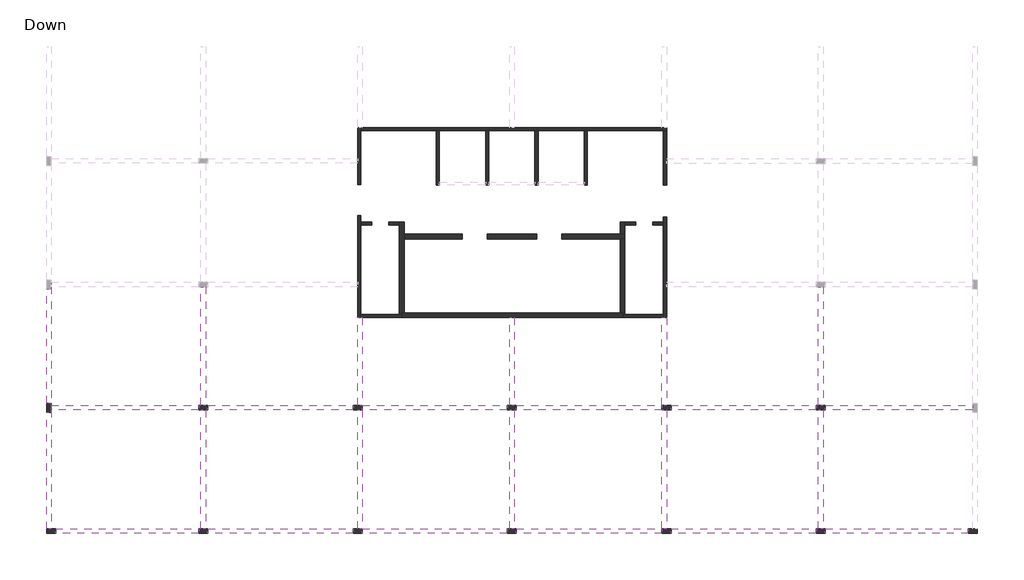
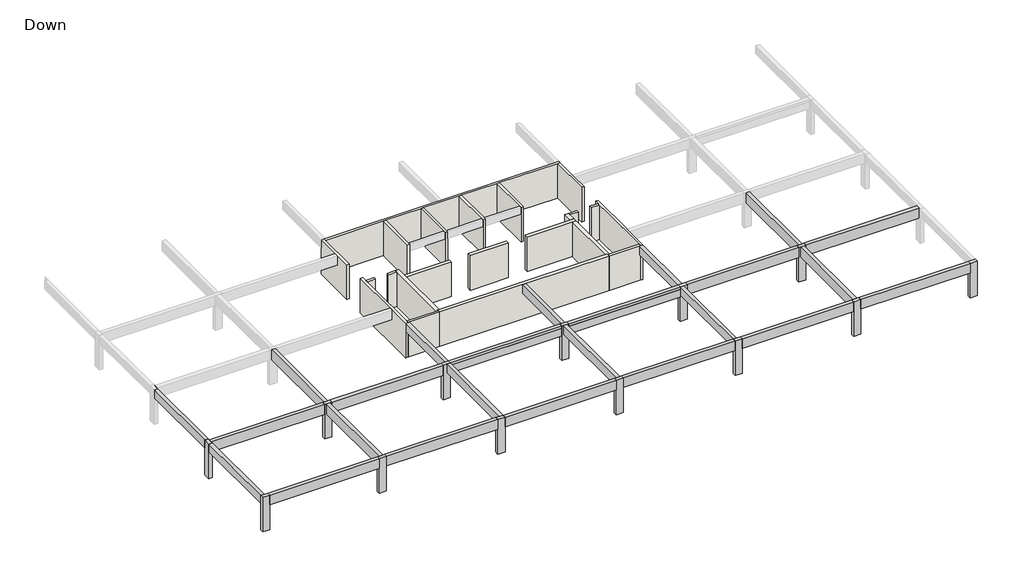
# One storey, part 1 of 2: 24 beams, 22 walls, 13 columns.
# Revit data of these elements (continued)
# Project information (continued)
#   Project Name = "Project 023"
#   Project Number = "מספר פרויקט"
# Type "Concrete Rectengular Beam : 30/70"
#   Length [instance default] = 152.4 cm
#   b = 30 cm
#   h = 70 cm
#   Structural Material [instance default] = Concrete
#   Assembly Code = ""
# Type "Concrete Rectengular Beam : 30/75"
#   Length [instance default] = 152.4 cm
#   b = 30 cm
#   h = 75 cm
#   Structural Material [instance default] = Concrete
#   Assembly Code = ""
# Type "Concrete Rectengular Beam : 30/85"
#   Length [instance default] = 152.4 cm
#   b = 30 cm
#   h = 85 cm
#   Structural Material [instance default] = Concrete
#   Assembly Code = ""
# Type "Concrete Rectengular Beam : 30/90"
#   Length [instance default] = 152.4 cm
#   b = 30 cm
#   h = 90 cm
#   Structural Material [instance default] = Concrete
#   Assembly Code = ""
# Type "Concrete Rectengular Column : 30/60"
#   b = 30 cm
#   h = 60 cm
#   Structural Material [instance default] = Concrete
# Type "20"
#   Layers, outside or top first: 20 cm "Concrete" (function 1)
# Type "30"
#   Layers, outside or top first: 30 cm "Concrete" (function 1)
# Element 1 (IfcBeam, "Concrete Rectengular Beam : 30/70")
#   Comments = ""
#   Mark = "B9"
#   SOFiSTiK_AMG_Comments = ""
#   SOFiSTiK_AMG_Scheduled = yes
#   SOFiSTiK_AMG_Adjusted = yes
#   Structural Material = Concrete
#   Phase Created = New Construction
#   Materials on its faces: "Concrete"
# Element 2 (IfcBeam, "Concrete Rectengular Beam : 30/70")
#   Comments = ""
#   Mark = "B10"
#   SOFiSTiK_AMG_Comments = ""
#   SOFiSTiK_AMG_Scheduled = yes
#   SOFiSTiK_AMG_Adjusted = yes
#   Structural Material = Concrete
#   Phase Created = New Construction
#   Materials on its faces: "Concrete"
# Element 3 (IfcBeam, "Concrete Rectengular Beam : 30/75")
#   Comments = ""
#   Mark = "B20"
#   SOFiSTiK_AMG_Comments = ""
#   SOFiSTiK_AMG_Scheduled = yes
#   SOFiSTiK_AMG_Adjusted = yes
#   Structural Material = Concrete
#   Phase Created = New Construction
#   Materials on its faces: "Concrete"
# Element 4 (IfcBeam, "Concrete Rectengular Beam : 30/75")
#   Comments = ""
#   Mark = "B21"
#   SOFiSTiK_AMG_Comments = ""
#   SOFiSTiK_AMG_Scheduled = yes
#   SOFiSTiK_AMG_Adjusted = yes
#   Structural Material = Concrete
#   Phase Created = New Construction
#   Materials on its faces: "Concrete"
# Element 5 (IfcBeam, "Concrete Rectengular Beam : 30/75")
#   Comments = ""
#   Mark = "B22"
#   SOFiSTiK_AMG_Comments = ""
#   SOFiSTiK_AMG_Scheduled = yes
#   SOFiSTiK_AMG_Adjusted = yes
#   Structural Material = Concrete
#   Phase Created = New Construction
#   Materials on its faces: "Concrete"
# Element 6 (IfcBeam, "Concrete Rectengular Beam : 30/75")
#   Comments = ""
#   Mark = "B23"
#   SOFiSTiK_AMG_Comments = ""
#   SOFiSTiK_AMG_Scheduled = yes
#   SOFiSTiK_AMG_Adjusted = yes
#   Structural Material = Concrete
#   Phase Created = New Construction
#   Materials on its faces: "Concrete"
# Element 7 (IfcBeam, "Concrete Rectengular Beam : 30/75")
#   Comments = ""
#   Mark = "B24"
#   SOFiSTiK_AMG_Comments = ""
#   SOFiSTiK_AMG_Scheduled = yes
#   SOFiSTiK_AMG_Adjusted = yes
#   Structural Material = Concrete
#   Phase Created = New Construction
#   Materials on its faces: "Concrete"
# Element 8 (IfcBeam, "Concrete Rectengular Beam : 30/75")
#   Comments = ""
#   Mark = "B25"
#   SOFiSTiK_AMG_Comments = ""
#   SOFiSTiK_AMG_Scheduled = yes
#   SOFiSTiK_AMG_Adjusted = yes
#   Structural Material = Concrete
#   Phase Created = New Construction
#   Materials on its faces: "Concrete"
# Element 9 (IfcBeam, "Concrete Rectengular Beam : 30/85")
#   Comments = ""
#   Mark = "B32"
#   SOFiSTiK_AMG_Comments = ""
#   SOFiSTiK_AMG_Scheduled = yes
#   SOFiSTiK_AMG_Adjusted = yes
#   Structural Material = Concrete
#   Phase Created = New Construction
#   Materials on its faces: "Concrete"
# Element 10 (IfcBeam, "Concrete Rectengular Beam : 30/85")
#   Comments = ""
#   Mark = "B33"
#   SOFiSTiK_AMG_Comments = ""
#   SOFiSTiK_AMG_Scheduled = yes
#   SOFiSTiK_AMG_Adjusted = yes
#   Structural Material = Concrete
#   Phase Created = New Construction
#   Materials on its faces: "Concrete"
# Element 11 (IfcBeam, "Concrete Rectengular Beam : 30/85")
#   Comments = ""
#   Mark = "B34"
#   SOFiSTiK_AMG_Comments = ""
#   SOFiSTiK_AMG_Scheduled = yes
#   SOFiSTiK_AMG_Adjusted = yes
#   Structural Material = Concrete
#   Phase Created = New Construction
#   Materials on its faces: "Concrete"
# Element 12 (IfcBeam, "Concrete Rectengular Beam : 30/85")
#   Comments = ""
#   Mark = "B35"
#   SOFiSTiK_AMG_Comments = ""
#   SOFiSTiK_AMG_Scheduled = yes
#   SOFiSTiK_AMG_Adjusted = yes
#   Structural Material = Concrete
#   Phase Created = New Construction
#   Materials on its faces: "Concrete"
# Element 13 (IfcBeam, "Concrete Rectengular Beam : 30/85")
#   Comments = ""
#   Mark = "B36"
#   SOFiSTiK_AMG_Comments = ""
#   SOFiSTiK_AMG_Scheduled = yes
#   SOFiSTiK_AMG_Adjusted = yes
#   Structural Material = Concrete
#   Phase Created = New Construction
#   Materials on its faces: "Concrete"
# Element 14 (IfcBeam, "Concrete Rectengular Beam : 30/85")
#   Comments = ""
#   Mark = "B37"
#   SOFiSTiK_AMG_Comments = ""
#   SOFiSTiK_AMG_Scheduled = yes
#   SOFiSTiK_AMG_Adjusted = yes
#   Structural Material = Concrete
#   Phase Created = New Construction
#   Materials on its faces: "Concrete"
# Element 15 (IfcBeam, "Concrete Rectengular Beam : 30/90")
#   Comments = ""
#   Mark = "B46"
#   SOFiSTiK_AMG_Comments = ""
#   SOFiSTiK_AMG_Scheduled = yes
#   SOFiSTiK_AMG_Adjusted = yes
#   Structural Material = Concrete
#   Phase Created = New Construction
#   Materials on its faces: "Concrete"
# Element 16 (IfcBeam, "Concrete Rectengular Beam : 30/90")
#   Comments = ""
#   Mark = "B47"
#   SOFiSTiK_AMG_Comments = ""
#   SOFiSTiK_AMG_Scheduled = yes
#   SOFiSTiK_AMG_Adjusted = yes
#   Structural Material = Concrete
#   Phase Created = New Construction
#   Materials on its faces: "Concrete"
# Element 17 (IfcBeam, "Concrete Rectengular Beam : 30/90")
#   Comments = ""
#   Mark = "B48"
#   SOFiSTiK_AMG_Comments = ""
#   SOFiSTiK_AMG_Scheduled = yes
#   SOFiSTiK_AMG_Adjusted = yes
#   Structural Material = Concrete
#   Phase Created = New Construction
#   Materials on its faces: "Concrete"
# Element 18 (IfcBeam, "Concrete Rectengular Beam : 30/90")
#   Comments = ""
#   Mark = "B49"
#   SOFiSTiK_AMG_Comments = ""
#   SOFiSTiK_AMG_Scheduled = yes
#   SOFiSTiK_AMG_Adjusted = yes
#   Structural Material = Concrete
#   Phase Created = New Construction
#   Materials on its faces: "Concrete"
# Element 19 (IfcBeam, "Concrete Rectengular Beam : 30/90")
#   Comments = ""
#   Mark = "B50"
#   SOFiSTiK_AMG_Comments = ""
#   SOFiSTiK_AMG_Scheduled = yes
#   SOFiSTiK_AMG_Adjusted = yes
#   Structural Material = Concrete
#   Phase Created = New Construction
#   Materials on its faces: "Concrete"
# Element 20 (IfcBeam, "Concrete Rectengular Beam : 30/90")
#   Comments = ""
#   Mark = "B51"
#   SOFiSTiK_AMG_Comments = ""
#   SOFiSTiK_AMG_Scheduled = yes
#   SOFiSTiK_AMG_Adjusted = yes
#   Structural Material = Concrete
#   Phase Created = New Construction
#   Materials on its faces: "Concrete"
# Element 21 (IfcBeam, "Concrete Rectengular Beam : 30/90")
#   Comments = ""
#   Mark = "B61"
#   SOFiSTiK_AMG_Comments = ""
#   SOFiSTiK_AMG_Scheduled = yes
#   SOFiSTiK_AMG_Adjusted = yes
#   Structural Material = Concrete
#   Phase Created = New Construction
#   Materials on its faces: "Concrete"
# Element 22 (IfcBeam, "Concrete Rectengular Beam : 30/90")
#   Comments = ""
#   Mark = "B62"
#   SOFiSTiK_AMG_Comments = ""
#   SOFiSTiK_AMG_Scheduled = yes
#   SOFiSTiK_AMG_Adjusted = yes
#   Structural Material = Concrete
#   Phase Created = New Construction
#   Materials on its faces: "Concrete"
# Element 23 (IfcBeam, "Concrete Rectengular Beam : 30/90")
#   Comments = ""
#   Mark = "B66"
#   SOFiSTiK_AMG_Comments = ""
#   SOFiSTiK_AMG_Scheduled = yes
#   SOFiSTiK_AMG_Adjusted = yes
#   Structural Material = Concrete
#   Phase Created = New Construction
#   Materials on its faces: "Concrete"
# Element 24 (IfcBeam, "Concrete Rectengular Beam : 30/90")
#   Comments = ""
#   Mark = "B67"
#   SOFiSTiK_AMG_Comments = ""
#   SOFiSTiK_AMG_Scheduled = yes
#   SOFiSTiK_AMG_Adjusted = yes
#   Structural Material = Concrete
#   Phase Created = New Construction
#   Materials on its faces: "Concrete"
# Element 25 (IfcColumn, "Concrete Rectengular Column : 30/60")
#   Comments = ""
#   Mark = "C3"
#   SOFiSTiK_AMG_Comments = ""
#   SOFiSTiK_AMG_Scheduled = yes
#   SOFiSTiK_AMG_Adjusted = yes
#   Structural Material = Concrete
#   Phase Created = New Construction
#   Materials on its faces: "Concrete"
# Element 26 (IfcColumn, "Concrete Rectengular Column : 30/60")
#   Comments = ""
#   Mark = "C7"
#   SOFiSTiK_AMG_Comments = ""
#   SOFiSTiK_AMG_Scheduled = yes
#   SOFiSTiK_AMG_Adjusted = yes
#   Structural Material = Concrete
#   Phase Created = New Construction
#   Materials on its faces: "Concrete"
# Element 27 (IfcColumn, "Concrete Rectengular Column : 30/60")
#   Comments = ""
#   Mark = "C8"
#   SOFiSTiK_AMG_Comments = ""
#   SOFiSTiK_AMG_Scheduled = yes
#   SOFiSTiK_AMG_Adjusted = yes
#   Structural Material = Concrete
#   Phase Created = New Construction
#   Materials on its faces: "Concrete"
# Element 28 (IfcColumn, "Concrete Rectengular Column : 30/60")
#   Comments = ""
#   Mark = "C14"
#   SOFiSTiK_AMG_Comments = ""
#   SOFiSTiK_AMG_Scheduled = yes
#   SOFiSTiK_AMG_Adjusted = yes
#   Structural Material = Concrete
#   Phase Created = New Construction
#   Materials on its faces: "Concrete"
# Element 29 (IfcColumn, "Concrete Rectengular Column : 30/60")
#   Comments = ""
#   Mark = "C15"
#   SOFiSTiK_AMG_Comments = ""
#   SOFiSTiK_AMG_Scheduled = yes
#   SOFiSTiK_AMG_Adjusted = yes
#   Structural Material = Concrete
#   Phase Created = New Construction
#   Materials on its faces: "Concrete"
# Element 30 (IfcColumn, "Concrete Rectengular Column : 30/60")
#   Comments = ""
#   Mark = "C17"
#   SOFiSTiK_AMG_Comments = ""
#   SOFiSTiK_AMG_Scheduled = yes
#   SOFiSTiK_AMG_Adjusted = yes
#   Structural Material = Concrete
#   Phase Created = New Construction
#   Materials on its faces: "Concrete"
# Element 31 (IfcColumn, "Concrete Rectengular Column : 30/60")
#   Comments = ""
#   Mark = "C23"
#   SOFiSTiK_AMG_Comments = ""
#   SOFiSTiK_AMG_Scheduled = yes
#   SOFiSTiK_AMG_Adjusted = yes
#   Structural Material = Concrete
#   Phase Created = New Construction
#   Materials on its faces: "Concrete"
# Element 32 (IfcColumn, "Concrete Rectengular Column : 30/60")
#   Comments = ""
#   Mark = "C24"
#   SOFiSTiK_AMG_Comments = ""
#   SOFiSTiK_AMG_Scheduled = yes
#   SOFiSTiK_AMG_Adjusted = yes
#   Structural Material = Concrete
#   Phase Created = New Construction
#   Materials on its faces: "Concrete"
# Element 33 (IfcColumn, "Concrete Rectengular Column : 30/60")
#   Comments = ""
#   Mark = "C25"
#   SOFiSTiK_AMG_Comments = ""
#   SOFiSTiK_AMG_Scheduled = yes
#   SOFiSTiK_AMG_Adjusted = yes
#   Structural Material = Concrete
#   Phase Created = New Construction
#   Materials on its faces: "Concrete"
# Element 34 (IfcColumn, "Concrete Rectengular Column : 30/60")
#   Comments = ""
#   Mark = "C26"
#   SOFiSTiK_AMG_Comments = ""
#   SOFiSTiK_AMG_Scheduled = yes
#   SOFiSTiK_AMG_Adjusted = yes
#   Structural Material = Concrete
#   Phase Created = New Construction
#   Materials on its faces: "Concrete"
# Element 35 (IfcColumn, "Concrete Rectengular Column : 30/60")
#   Comments = ""
#   Mark = "C27"
#   SOFiSTiK_AMG_Comments = ""
#   SOFiSTiK_AMG_Scheduled = yes
#   SOFiSTiK_AMG_Adjusted = yes
#   Structural Material = Concrete
#   Phase Created = New Construction
#   Materials on its faces: "Concrete"
# Element 36 (IfcColumn, "Concrete Rectengular Column : 30/60")
#   Comments = ""
#   Mark = "C35"
#   SOFiSTiK_AMG_Comments = ""
#   SOFiSTiK_AMG_Scheduled = yes
#   SOFiSTiK_AMG_Adjusted = yes
#   Structural Material = Concrete
#   Phase Created = New Construction
#   Materials on its faces: "Concrete"
# Element 37 (IfcColumn, "Concrete Rectengular Column : 30/60")
#   Comments = ""
#   Mark = "C36"
#   SOFiSTiK_AMG_Comments = ""
#   SOFiSTiK_AMG_Scheduled = yes
#   SOFiSTiK_AMG_Adjusted = yes
#   Structural Material = Concrete
#   Phase Created = New Construction
#   Materials on its faces: "Concrete"
# Element 38 (IfcWall, "20")
#   Comments = ""
#   Mark = "W1"
#   SOFiSTiK_EdgeZones = "W1"
#   SOFiSTiK_AMG_Comments = ""
#   Top Offset = 0 cm
#   Base Offset = 0 cm
#   wall height = 308 cm
#   SOFiSTiK_AMG_Scheduled = yes
#   SOFiSTiK_AMG_Adjusted = yes
#   Phase Created = New Construction
#   Base Constraint = Down
#   Top Constraint = Typical Floor
#   Materials on its faces: "Concrete"
# Element 39 (IfcWall, "20")
#   Comments = ""
#   Mark = "W2"
#   SOFiSTiK_EdgeZones = "W2"
#   SOFiSTiK_AMG_Comments = ""
#   Top Offset = 0 cm
#   Base Offset = 0 cm
#   wall height = 308 cm
#   SOFiSTiK_AMG_Scheduled = yes
#   SOFiSTiK_AMG_Adjusted = yes
#   Phase Created = New Construction
#   Base Constraint = Down
#   Top Constraint = Typical Floor
#   Materials on its faces: "Concrete"
# Element 40 (IfcWall, "20")
#   Comments = ""
#   Mark = "W3"
#   SOFiSTiK_EdgeZones = "W3"
#   SOFiSTiK_AMG_Comments = ""
#   Top Offset = 0 cm
#   Base Offset = 0 cm
#   wall height = 308 cm
#   SOFiSTiK_AMG_Scheduled = yes
#   SOFiSTiK_AMG_Adjusted = yes
#   Phase Created = New Construction
#   Base Constraint = Down
#   Top Constraint = Typical Floor
#   Materials on its faces: "Concrete"
# Element 41 (IfcWall, "20")
#   Comments = ""
#   Mark = "W4"
#   SOFiSTiK_EdgeZones = "W4"
#   SOFiSTiK_AMG_Comments = ""
#   Top Offset = 0 cm
#   Base Offset = 0 cm
#   wall height = 308 cm
#   SOFiSTiK_AMG_Scheduled = yes
#   SOFiSTiK_AMG_Adjusted = yes
#   Phase Created = New Construction
#   Base Constraint = Down
#   Top Constraint = Typical Floor
#   Materials on its faces: "Concrete"
# Element 42 (IfcWall, "20")
#   Comments = ""
#   Mark = "W5"
#   SOFiSTiK_EdgeZones = "W5"
#   SOFiSTiK_AMG_Comments = ""
#   Top Offset = 0 cm
#   Base Offset = 0 cm
#   wall height = 308 cm
#   SOFiSTiK_AMG_Scheduled = yes
#   SOFiSTiK_AMG_Adjusted = yes
#   Phase Created = New Construction
#   Base Constraint = Down
#   Top Constraint = Typical Floor
#   Materials on its faces: "Concrete"
# Element 43 (IfcWall, "20")
#   Comments = ""
#   Mark = "W6"
#   SOFiSTiK_EdgeZones = "W6"
#   SOFiSTiK_AMG_Comments = ""
#   Top Offset = 0 cm
#   Base Offset = 0 cm
#   wall height = 308 cm
#   SOFiSTiK_AMG_Scheduled = yes
#   SOFiSTiK_AMG_Adjusted = yes
#   Phase Created = New Construction
#   Base Constraint = Down
#   Top Constraint = Typical Floor
#   Materials on its faces: "Concrete"
# Element 44 (IfcWall, "20")
#   Comments = ""
#   Mark = "W7"
#   SOFiSTiK_EdgeZones = "W7"
#   SOFiSTiK_AMG_Comments = ""
#   Top Offset = 0 cm
#   Base Offset = 0 cm
#   wall height = 308 cm
#   SOFiSTiK_AMG_Scheduled = yes
#   SOFiSTiK_AMG_Adjusted = yes
#   Phase Created = New Construction
#   Base Constraint = Down
#   Top Constraint = Typical Floor
#   Materials on its faces: "Concrete"
# Element 45 (IfcWall, "20")
#   Comments = ""
#   Mark = "W8"
#   SOFiSTiK_EdgeZones = "W8"
#   SOFiSTiK_AMG_Comments = ""
#   Top Offset = 0 cm
#   Base Offset = 0 cm
#   wall height = 308 cm
#   SOFiSTiK_AMG_Scheduled = yes
#   SOFiSTiK_AMG_Adjusted = yes
#   Phase Created = New Construction
#   Base Constraint = Down
#   Top Constraint = Typical Floor
#   Materials on its faces: "Concrete"
# Element 46 (IfcWall, "20")
#   Comments = ""
#   Mark = "W9"
#   SOFiSTiK_EdgeZones = "W9"
#   SOFiSTiK_AMG_Comments = ""
#   Top Offset = 0 cm
#   Base Offset = 0 cm
#   wall height = 308 cm
#   SOFiSTiK_AMG_Scheduled = yes
#   SOFiSTiK_AMG_Adjusted = yes
#   Phase Created = New Construction
#   Base Constraint = Down
#   Top Constraint = Typical Floor
#   Materials on its faces: "Concrete"
# Element 47 (IfcWall, "20")
#   Comments = ""
#   Mark = "W10"
#   SOFiSTiK_EdgeZones = "W10"
#   SOFiSTiK_AMG_Comments = ""
#   Top Offset = 0 cm
#   Base Offset = 0 cm
#   wall height = 308 cm
#   SOFiSTiK_AMG_Scheduled = yes
#   SOFiSTiK_AMG_Adjusted = yes
#   Phase Created = New Construction
#   Base Constraint = Down
#   Top Constraint = Typical Floor
#   Materials on its faces: "Concrete"
# Element 48 (IfcWall, "20")
#   Comments = ""
#   Mark = "W11"
#   SOFiSTiK_EdgeZones = "W11"
#   SOFiSTiK_AMG_Comments = ""
#   Top Offset = 0 cm
#   Base Offset = 0 cm
#   wall height = 308 cm
#   SOFiSTiK_AMG_Scheduled = yes
#   SOFiSTiK_AMG_Adjusted = yes
#   Phase Created = New Construction
#   Base Constraint = Down
#   Top Constraint = Typical Floor
#   Materials on its faces: "Concrete"
# Element 49 (IfcWall, "20")
#   Comments = ""
#   Mark = "W12"
#   SOFiSTiK_EdgeZones = "W12"
#   SOFiSTiK_AMG_Comments = ""
#   Top Offset = 0 cm
#   Base Offset = 0 cm
#   wall height = 308 cm
#   SOFiSTiK_AMG_Scheduled = yes
#   SOFiSTiK_AMG_Adjusted = yes
#   Phase Created = New Construction
#   Base Constraint = Down
#   Top Constraint = Typical Floor
#   Materials on its faces: "Concrete"
# Element 50 (IfcWall, "20")
#   Comments = ""
#   Mark = "W13"
#   SOFiSTiK_EdgeZones = "W13"
#   SOFiSTiK_AMG_Comments = ""
#   Top Offset = 0 cm
#   Base Offset = 0 cm
#   wall height = 308 cm
#   SOFiSTiK_AMG_Scheduled = yes
#   SOFiSTiK_AMG_Adjusted = yes
#   Phase Created = New Construction
#   Base Constraint = Down
#   Top Constraint = Typical Floor
#   Materials on its faces: "Concrete"
# Element 51 (IfcWall, "20")
#   Comments = ""
#   Mark = "W14"
#   SOFiSTiK_EdgeZones = "W14"
#   SOFiSTiK_AMG_Comments = ""
#   Top Offset = 0 cm
#   Base Offset = 0 cm
#   wall height = 308 cm
#   SOFiSTiK_AMG_Scheduled = yes
#   SOFiSTiK_AMG_Adjusted = yes
#   Phase Created = New Construction
#   Base Constraint = Down
#   Top Constraint = Typical Floor
#   Materials on its faces: "Concrete"
# Element 52 (IfcWall, "20")
#   Comments = ""
#   Mark = "W15"
#   SOFiSTiK_EdgeZones = "W15"
#   SOFiSTiK_AMG_Comments = ""
#   Top Offset = 0 cm
#   Base Offset = 0 cm
#   wall height = 308 cm
#   SOFiSTiK_AMG_Scheduled = yes
#   SOFiSTiK_AMG_Adjusted = yes
#   Phase Created = New Construction
#   Base Constraint = Down
#   Top Constraint = Typical Floor
#   Materials on its faces: "Concrete"
# Element 53 (IfcWall, "30")
#   Comments = ""
#   Mark = "W16"
#   SOFiSTiK_EdgeZones = "W16"
#   SOFiSTiK_AMG_Comments = ""
#   Top Offset = 0 cm
#   Base Offset = 0 cm
#   wall height = 308 cm
#   SOFiSTiK_AMG_Scheduled = yes
#   SOFiSTiK_AMG_Adjusted = yes
#   Phase Created = New Construction
#   Base Constraint = Down
#   Top Constraint = Typical Floor
#   Materials on its faces: "Concrete"
# Element 54 (IfcWall, "30")
#   Comments = ""
#   Mark = "W17"
#   SOFiSTiK_EdgeZones = "W17"
#   SOFiSTiK_AMG_Comments = ""
#   Top Offset = 0 cm
#   Base Offset = 0 cm
#   wall height = 308 cm
#   SOFiSTiK_AMG_Scheduled = yes
#   SOFiSTiK_AMG_Adjusted = yes
#   Phase Created = New Construction
#   Base Constraint = Down
#   Top Constraint = Typical Floor
#   Materials on its faces: "Concrete"
# Element 55 (IfcWall, "30")
#   Comments = ""
#   Mark = "W18"
#   SOFiSTiK_EdgeZones = "W18"
#   SOFiSTiK_AMG_Comments = ""
#   Top Offset = 0 cm
#   Base Offset = 0 cm
#   wall height = 308 cm
#   SOFiSTiK_AMG_Scheduled = yes
#   SOFiSTiK_AMG_Adjusted = yes
#   Phase Created = New Construction
#   Base Constraint = Down
#   Top Constraint = Typical Floor
#   Materials on its faces: "Concrete"
# Element 56 (IfcWall, "30")
#   Comments = ""
#   Mark = "W19"
#   SOFiSTiK_EdgeZones = "W19"
#   SOFiSTiK_AMG_Comments = ""
#   Top Offset = 0 cm
#   Base Offset = 0 cm
#   wall height = 308 cm
#   SOFiSTiK_AMG_Scheduled = yes
#   SOFiSTiK_AMG_Adjusted = yes
#   Phase Created = New Construction
#   Base Constraint = Down
#   Top Constraint = Typical Floor
#   Materials on its faces: "Concrete"
# Element 57 (IfcWall, "30")
#   Comments = ""
#   Mark = "W20"
#   SOFiSTiK_EdgeZones = "W20"
#   SOFiSTiK_AMG_Comments = ""
#   Top Offset = 0 cm
#   Base Offset = 0 cm
#   wall height = 308 cm
#   SOFiSTiK_AMG_Scheduled = yes
#   SOFiSTiK_AMG_Adjusted = yes
#   Phase Created = New Construction
#   Base Constraint = Down
#   Top Constraint = Typical Floor
#   Materials on its faces: "Concrete"
# Element 58 (IfcWall, "30")
#   Comments = ""
#   Mark = "W21"
#   SOFiSTiK_EdgeZones = "W21"
#   SOFiSTiK_AMG_Comments = ""
#   Top Offset = 0 cm
#   Base Offset = 0 cm
#   wall height = 308 cm
#   SOFiSTiK_AMG_Scheduled = yes
#   SOFiSTiK_AMG_Adjusted = yes
#   Phase Created = New Construction
#   Base Constraint = Down
#   Top Constraint = Typical Floor
#   Materials on its faces: "Concrete"
# Element 59 (IfcWall, "30")
#   Comments = ""
#   Mark = "W22"
#   SOFiSTiK_EdgeZones = "W22"
#   SOFiSTiK_AMG_Comments = ""
#   Top Offset = 0 cm
#   Base Offset = 0 cm
#   wall height = 308 cm
#   SOFiSTiK_AMG_Scheduled = yes
#   SOFiSTiK_AMG_Adjusted = yes
#   Phase Created = New Construction
#   Base Constraint = Down
#   Top Constraint = Typical Floor
#   Materials on its faces: "Concrete"
# Materials
#   "Concrete": class "Concrete", colour RGB 192 192 192, transparency 0, Keynote = "01000", Description = "Cast-in-place concrete", Cost = 0
